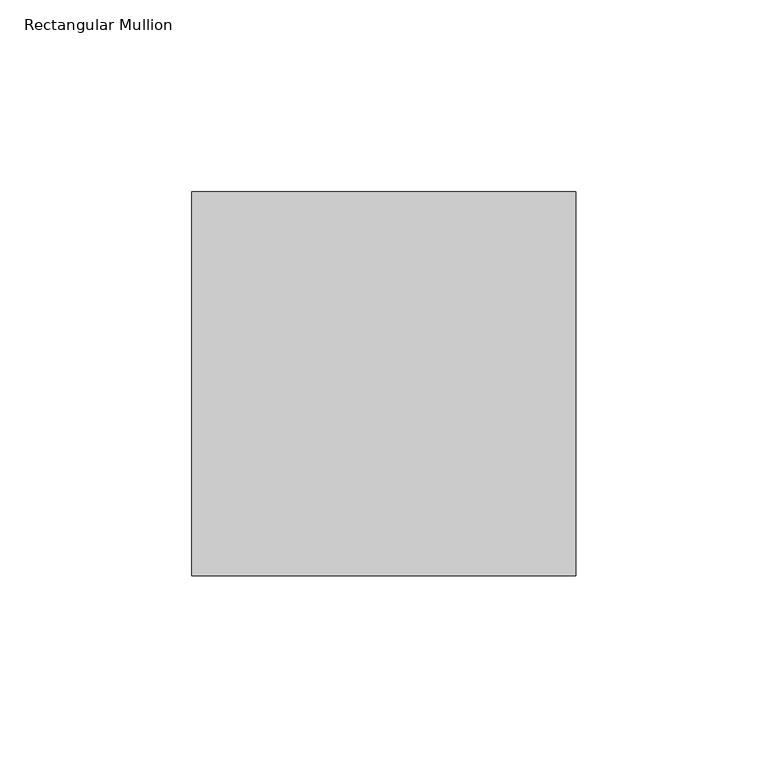
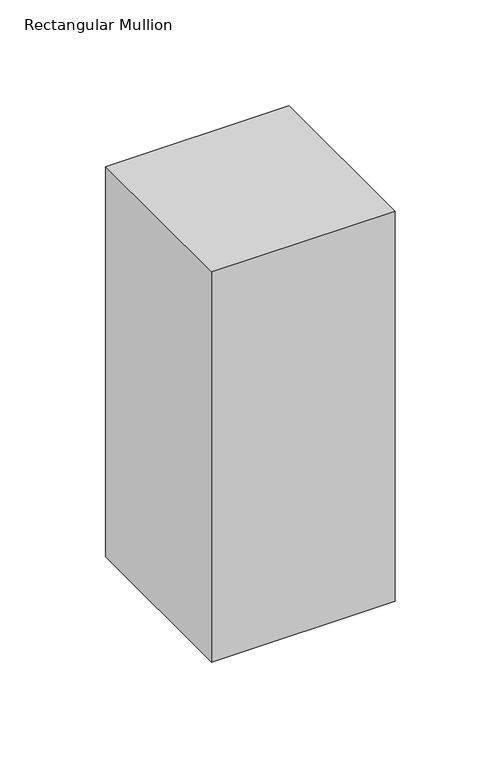
"""IFC4 building model written with IfcOpenShell, lengths in millimetres: member geometry, Rectangular Mullion : 알루미늄_Rectangular Cap_100 x100."""

from ifc_helpers import new_model, si_unit, frame, origin, place, context, project, spatial, polyline, outline, extrude, source, transform, mapped, element, save


def rectangular_mullion_f7ac6ae7(model_context):
    return source(origin(), model_context, "Body", "SweptSolid", [
        extrude(outline(polyline([(0.0, 50.0), (0.0, -50.0), (-100.0, -50.0), (-100.0, 50.0), (0.0, 50.0)])), frame((0.0, 0.0, -225.0), z_axis=(0.0, 0.0, 1.0), x_axis=(1.0, 0.0, 0.0)), (0.0, 0.0, 1.0), 225.0),
    ])


if __name__ == "__main__":
    model = new_model("IFC4")
    model_context = context("Model", 3, world=origin())
    ifc_project = project(units=[si_unit("LENGTHUNIT", "METRE", prefix="MILLI")], contexts=[model_context])
    site = spatial("IfcSite", under=ifc_project)
    building = spatial("IfcBuilding", under=site)
    placement = place(None, origin())
    rectangular_mullion_shape = rectangular_mullion_f7ac6ae7(model_context)
    element("IfcMember", 1, ObjectType="Rectangular Mullion : 알루미늄_Rectangular Cap_100 x100", at=placement, inside=building, context=model_context, shape_type="MappedRepresentation", body=[
        mapped(rectangular_mullion_shape, transform((0.0, 0.0, 0.0), x_axis=(1.0, 0.0, 0.0), y_axis=(0.0, 1.0, 0.0), z_axis=(0.0, 0.0, 1.0))),
    ])
    save(model, "model.ifc")

# Revit data of these elements
# Type "Rectangular Mullion : 알루미늄_Rectangular Cap_100 x100"
#   built-in parameter 1007304 = 0.328084 (stored number, unit not read)
#   built-in parameter 1007301 = 0.164042 (stored number, unit not read)
#   built-in parameter 1007300 = 0.164042 (stored number, unit not read)
# Element 1 (IfcMember, "Rectangular Mullion : 알루미늄_Rectangular Cap_100 x100")
#   Materials on its faces: "00_Metal_Stainless Steel"
# Materials
#   "00_Metal_Stainless Steel": class "Metal", colour RGB 148 148 148, transparency 0, Description = "Steel", Cost = 0
